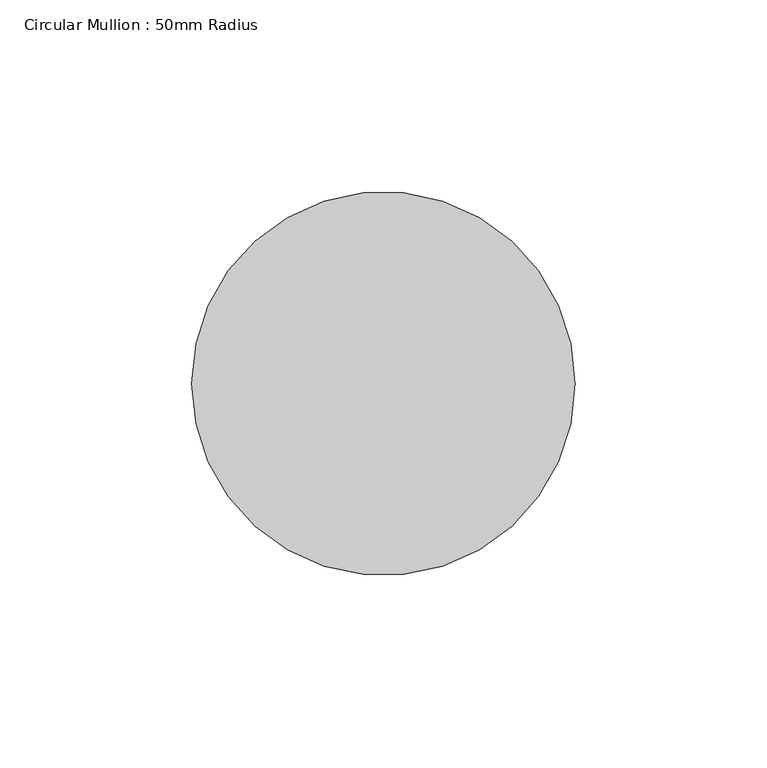
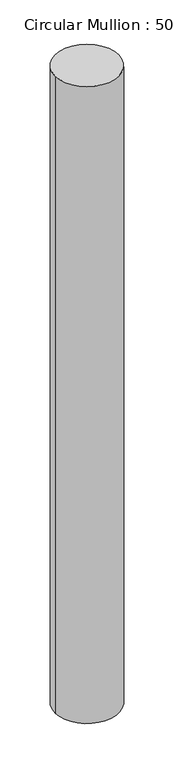
"""IFC4 building model written with IfcOpenShell, lengths in millimetres: member geometry, Circular Mullion : 50mm Radius."""

from ifc_helpers import new_model, si_unit, point, frame, origin, origin_2d, place, context, project, spatial, circle_curve, trimmed, segment, composite_curve, outline, extrude, source, transform, mapped, element, save


def circular_mullion_50mm_radius_59ae8acb(model_context):
    return source(origin(), model_context, "Body", "SweptSolid", [
        extrude(outline(composite_curve([segment(trimmed(circle_curve(origin_2d(), 50.0), [point((50.0, 0.0))], [point((-50.0, 0.0))], False, "CARTESIAN"), True, "CONTINUOUS"), segment(trimmed(circle_curve(origin_2d(), 50.0), [point((-50.0, 0.0))], [point((50.0, 0.0))], False, "CARTESIAN"), True, "CONTINUOUS")], self_intersect=False)), frame((0.0, 0.0, -1058.4640831), z_axis=(0.0, 0.0, 1.0), x_axis=(1.0, 0.0, 0.0)), (0.0, 0.0, 1.0), 1058.4640831),
    ])


if __name__ == "__main__":
    model = new_model("IFC4")
    model_context = context("Model", 3, world=origin())
    ifc_project = project(units=[si_unit("LENGTHUNIT", "METRE", prefix="MILLI")], contexts=[model_context])
    site = spatial("IfcSite", under=ifc_project)
    building = spatial("IfcBuilding", under=site)
    placement = place(None, origin())
    circular_mullion_50mm_radius_shape = circular_mullion_50mm_radius_59ae8acb(model_context)
    element("IfcMember", 1, ObjectType="Circular Mullion : 50mm Radius", at=placement, inside=building, context=model_context, shape_type="MappedRepresentation", body=[
        mapped(circular_mullion_50mm_radius_shape, transform((0.0, 0.0, 0.0), x_axis=(1.0, 0.0, 0.0), y_axis=(0.0, 1.0, 0.0), z_axis=(0.0, 0.0, 1.0))),
    ])
    save(model, "model.ifc")

# Revit data of these elements
# Type "Circular Mullion : 50mm Radius"
#   built-in parameter 1007350 = 0.164042 (stored number, unit not read)
# Element 1 (IfcMember, "Circular Mullion : 50mm Radius")
#   Materials on its faces: "Aluminium"
# Materials
#   "Aluminium": class "Metal", colour RGB 247 247 247, transparency 0, Description = "Aluminium 6061", Cost = 0
